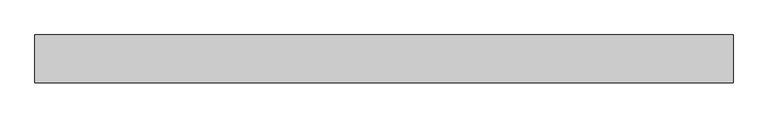
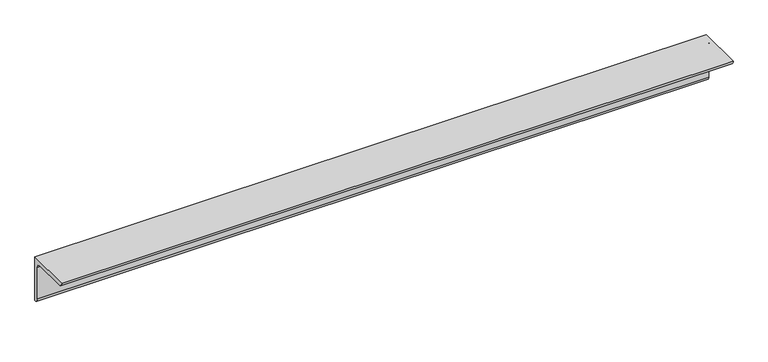
"""IFC4 building model written with IfcOpenShell, lengths in millimetres: member geometry, 0912_Steel Framing_L-KSD3502 : H_SB_AR_S03_L-130x130x12_HBR3."""

from ifc_helpers import new_model, si_unit, point, frame, frame_2d, origin, place, context, project, spatial, polyline, circle_curve, trimmed, segment, composite_curve, outline, extrude, source, transform, mapped, element, save


def member_eefd757e(model_context):
    return source(origin(), model_context, "Body", "SweptSolid", [
        extrude(outline(composite_curve([segment(polyline([(36.4, 36.4), (36.4, -93.6)]), True, "CONTINUOUS"), segment(trimmed(circle_curve(frame_2d((36.4, -81.6)), 12.0), [point((36.4, -93.6))], [point((24.4, -81.6))], False, "CARTESIAN"), True, "CONTINUOUS"), segment(polyline([(24.4, -81.6), (24.4, 12.4)]), True, "CONTINUOUS"), segment(trimmed(circle_curve(frame_2d((12.4, 12.4)), 12.0), [point((24.4, 12.4))], [point((12.4, 24.4))], True, "CARTESIAN"), True, "CONTINUOUS"), segment(polyline([(12.4, 24.4), (-81.6, 24.4)]), True, "CONTINUOUS"), segment(trimmed(circle_curve(frame_2d((-81.6, 36.4)), 12.0), [point((-81.6, 24.4))], [point((-93.6, 36.4))], False, "CARTESIAN"), True, "CONTINUOUS"), segment(polyline([(-93.6, 36.4), (36.4, 36.4)]), True, "CONTINUOUS")], self_intersect=False)), frame((-885.3576412, 0.0, 0.0), z_axis=(1.0, 0.0, 0.0), x_axis=(0.0, 1.0, 0.0)), (0.0, 0.0, 1.0), 1889.881949),
    ])


if __name__ == "__main__":
    model = new_model("IFC4")
    model_context = context("Model", 3, world=origin())
    ifc_project = project(units=[si_unit("LENGTHUNIT", "METRE", prefix="MILLI")], contexts=[model_context])
    site = spatial("IfcSite", under=ifc_project)
    building = spatial("IfcBuilding", under=site)
    placement = place(None, origin())
    member_shape = member_eefd757e(model_context)
    element("IfcMember", 1, ObjectType="0912_Steel Framing_L-KSD3502 : H_SB_AR_S03_L-130x130x12_HBR3", at=placement, inside=building, context=model_context, shape_type="MappedRepresentation", body=[
        mapped(member_shape, transform((0.0, 0.0, 0.0), x_axis=(1.0, 0.0, 0.0), y_axis=(0.0, 1.0, 0.0), z_axis=(0.0, 0.0, 1.0))),
    ])
    save(model, "model.ifc")

# Revit data of these elements
# Type "0912_Steel Framing_L-KSD3502 : H_SB_AR_S03_L-130x130x12_HBR3"
#   k = 25 mm
#   Perimeter = 0.52 m²/m
#   Nominal Weight = 23.40 kgf/m
#   Length [instance default] = 1000 mm
#   b = 130 mm
#   d = 130 mm
#   t = 12 mm
#   x = 36.4 mm
#   y = 36.4 mm
#   A = 2976.00 m²
#   Structural Material [instance default] = Steel, 45-345
# Element 1 (IfcMember, "0912_Steel Framing_L-KSD3502 : H_SB_AR_S03_L-130x130x12_HBR3")
#   Materials on its faces: "Steel, 45-345"
# Materials
#   "Steel, 45-345": class "Metal", colour RGB 189 187 185, transparency 0, Description = "Steel 345 MPa", Cost = 0
